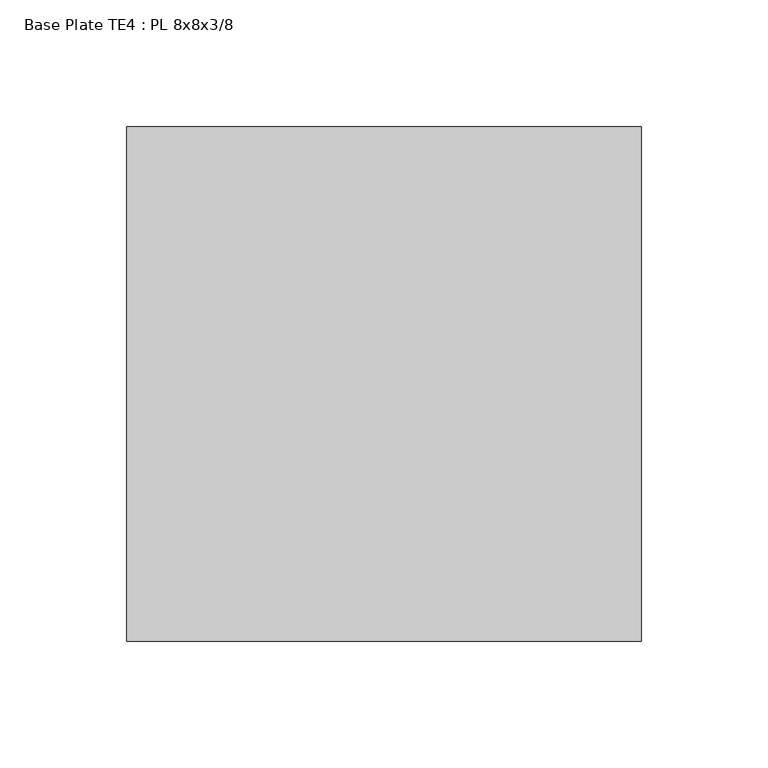
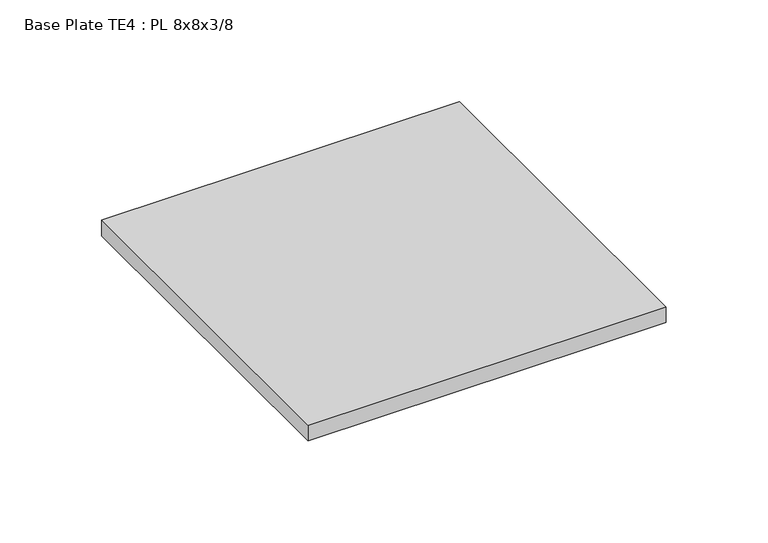
"""IFC4 building model written with IfcOpenShell, lengths in millimetres: proxy geometry, Base Plate TE4 : PL 8x8x3/8."""

import ifcopenshell
import ifcopenshell.guid

model = None  # the IFC model being written
_history = None  # IfcOwnerHistory: only IFC2X3 demands one
_inside = {}  # id of a spatial element -> (the spatial element, [elements in it])
_under = {}  # id of a project, library or spatial element -> (it, [spatial elements below it])
_declared = {}  # id of a project -> (the project, [libraries it declares])
_typed = {}  # id of a type object -> (the type object, [elements of that type])
_made_of = {}  # id of a material, layer set ... -> (it, [elements and type objects made of it])


def new_model(schema):
    """Start an empty IFC model of exactly this schema.

    Asked for "IFC4X3", IfcOpenShell would pick the latest addendum, in which some entities
    have other attributes; the version numbers below select the first issue.
    IFC2X3 requires an IfcOwnerHistory on every rooted entity: one is made here for all.
    """
    global model, _history
    if schema == "IFC4X3":
        model = ifcopenshell.file(schema_version=(4, 3, 0, 0))
    else:
        model = ifcopenshell.file(schema=schema)
    _inside.clear()
    _under.clear()
    _declared.clear()
    _typed.clear()
    _made_of.clear()
    _history = None
    if model.schema == "IFC2X3":
        org = make("IfcOrganization", Name="unknown")
        user = make(
            "IfcPersonAndOrganization",
            ThePerson=make("IfcPerson", FamilyName="unknown"),
            TheOrganization=org,
        )
        app = make(
            "IfcApplication",
            ApplicationDeveloper=org,
            Version="unknown",
            ApplicationFullName="unknown",
            ApplicationIdentifier="unknown",
        )
        _history = make(
            "IfcOwnerHistory",
            OwningUser=user,
            OwningApplication=app,
            ChangeAction="ADDED",
            CreationDate=0,
        )
    return model


def make(cls, **values):
    """One entity of the class cls with the attributes given. An attribute that is None is left unset."""
    return model.create_entity(
        cls, **{name: value for name, value in values.items() if value is not None}
    )


def rooted(cls, **values):
    """An entity with a GlobalId (a new one), such as an element, a storey or a relation."""
    return make(cls, GlobalId=ifcopenshell.guid.new(), OwnerHistory=_history, **values)


def si_unit(unit_type, name, prefix=None):
    """IfcSIUnit, for example si_unit("LENGTHUNIT", "METRE", prefix="MILLI")."""
    return make("IfcSIUnit", UnitType=unit_type, Prefix=prefix, Name=name)


def assignment(units):
    """IfcUnitAssignment: the units of a project."""
    return None if units is None else make("IfcUnitAssignment", Units=units)


def point(xyz):
    """IfcCartesianPoint."""
    return None if xyz is None else make("IfcCartesianPoint", Coordinates=xyz)


def direction(xyz):
    """IfcDirection."""
    return None if xyz is None else make("IfcDirection", DirectionRatios=xyz)


def frame(location, z_axis=None, x_axis=None):
    """IfcAxis2Placement3D, a coordinate frame: its origin and axes. An axis left out is left unset."""
    return make(
        "IfcAxis2Placement3D",
        Location=point(location),
        Axis=direction(z_axis),
        RefDirection=direction(x_axis),
    )


def origin():
    """The frame at (0, 0, 0) with its axes left unset."""
    return frame((0.0, 0.0, 0.0))


def place(relative_to, where):
    """IfcLocalPlacement: puts the frame where relative to a parent placement (None: the world)."""
    return make(
        "IfcLocalPlacement", PlacementRelTo=relative_to, RelativePlacement=where
    )


def context(
    kind, dimensions, precision=None, world=None, true_north=None, identifier=None
):
    """IfcGeometricRepresentationContext, for example the 3D "Model" context."""
    return make(
        "IfcGeometricRepresentationContext",
        ContextIdentifier=identifier,
        ContextType=kind,
        CoordinateSpaceDimension=dimensions,
        Precision=precision,
        WorldCoordinateSystem=world,
        TrueNorth=true_north,
    )


def project(units=None, contexts=None):
    """IfcProject with its units and contexts."""
    return rooted(
        "IfcProject",
        Name="project",
        RepresentationContexts=contexts,
        UnitsInContext=assignment(units),
    )


def spatial(cls, under=None, at=None, **own):
    """A site, building, storey or space (cls), placed at a placement, below another one or the project."""
    s = rooted(cls, ObjectPlacement=at, **own)
    if under is not None:
        _under.setdefault(under.id(), (under, []))[1].append(s)
    return s


def polyline(points):
    """IfcPolyline through the points."""
    return make("IfcPolyline", Points=[point(p) for p in points])


def outline(outer, holes=None, kind="AREA"):
    """IfcArbitraryClosedProfileDef: a profile drawn as a closed curve; with holes, ...WithVoids."""
    if holes is None:
        return make("IfcArbitraryClosedProfileDef", ProfileType=kind, OuterCurve=outer)
    return make(
        "IfcArbitraryProfileDefWithVoids",
        ProfileType=kind,
        OuterCurve=outer,
        InnerCurves=holes,
    )


def extrude(swept, where, along, depth):
    """IfcExtrudedAreaSolid: the profile swept, set in the frame where, extruded along a direction by depth."""
    return make(
        "IfcExtrudedAreaSolid",
        SweptArea=swept,
        Position=where,
        ExtrudedDirection=direction(along),
        Depth=depth,
    )


def shape(context_of_items, identifier, shape_type, items):
    """IfcShapeRepresentation: the items that make up one representation, for example the "Body"."""
    return make(
        "IfcShapeRepresentation",
        ContextOfItems=context_of_items,
        RepresentationIdentifier=identifier,
        RepresentationType=shape_type,
        Items=items,
    )


def source(mapping_origin, context_of_items, identifier, shape_type, items):
    """IfcRepresentationMap: a shape defined once, which mapped items show again and again."""
    return make(
        "IfcRepresentationMap",
        MappingOrigin=mapping_origin,
        MappedRepresentation=shape(context_of_items, identifier, shape_type, items),
    )


def transform(
    local_origin,
    x_axis=None,
    y_axis=None,
    z_axis=None,
    scale=None,
    scale2=None,
    scale3=None,
    uniform=True,
):
    """IfcCartesianTransformationOperator3D, or its non-uniform kind. x_axis, y_axis, z_axis: its Axis1, 2, 3."""
    if uniform:
        return make(
            "IfcCartesianTransformationOperator3D",
            Axis1=direction(x_axis),
            Axis2=direction(y_axis),
            LocalOrigin=point(local_origin),
            Scale=scale,
            Axis3=direction(z_axis),
        )
    return make(
        "IfcCartesianTransformationOperator3DnonUniform",
        Axis1=direction(x_axis),
        Axis2=direction(y_axis),
        LocalOrigin=point(local_origin),
        Scale=scale,
        Axis3=direction(z_axis),
        Scale2=scale2,
        Scale3=scale3,
    )


def mapped(mapping_source, mapping_target):
    """IfcMappedItem: shows the shape of a source again, moved by a transform."""
    return make(
        "IfcMappedItem", MappingSource=mapping_source, MappingTarget=mapping_target
    )


def made_of(thing, what):
    """Note that an element or type object is made of a material, layer set ...; save() writes the relation."""
    if what is not None:
        _made_of.setdefault(what.id(), (what, []))[1].append(thing)
    return thing


def element(
    cls,
    number,
    at=None,
    inside=None,
    cuts=None,
    type_object=None,
    material=None,
    context=None,
    identifier="Body",
    shape_type=None,
    held_by="IfcProductDefinitionShape",
    body=None,
    shapes=None,
    **own,
):
    """One element of the class cls, such as IfcWall. Its Tag is "e" and its number.

    at: its placement. inside: the storey or other place that contains it. cuts: it is an
    opening in that element (IfcRelVoidsElement). A single representation is given by context,
    identifier, shape_type and body (its items); several are given by shapes. held_by: the class
    of the entity that holds the representations. save() writes the other relations.
    """
    e = rooted(cls, Tag="e%d" % number, ObjectPlacement=at, **own)
    if body is not None:
        shapes = [shape(context, identifier, shape_type, body)]
    if shapes is not None:
        e.Representation = make(held_by, Representations=shapes)
    if inside is not None:
        _inside.setdefault(inside.id(), (inside, []))[1].append(e)
    if cuts is not None:
        rooted(
            "IfcRelVoidsElement", RelatingBuildingElement=cuts, RelatedOpeningElement=e
        )
    if type_object is not None:
        _typed.setdefault(type_object.id(), (type_object, []))[1].append(e)
    return made_of(e, material)


def aggregate(whole, parts):
    """IfcRelAggregates: a whole, such as a stair, and the parts it consists of."""
    return rooted("IfcRelAggregates", RelatingObject=whole, RelatedObjects=parts)


def save(model, path):
    """Write the relations noted so far, then the file.

    IfcRelAggregates (storeys below a building ...), IfcRelContainedInSpatialStructure (elements
    in a storey), IfcRelDefinesByType, IfcRelAssociatesMaterial and IfcRelDeclares: one each for
    every whole, place, type object, material and project.
    """
    for whole, parts in _under.values():
        aggregate(whole, parts)
    for where, things in _inside.values():
        rooted(
            "IfcRelContainedInSpatialStructure",
            RelatedElements=things,
            RelatingStructure=where,
        )
    for kind, things in _typed.values():
        rooted("IfcRelDefinesByType", RelatedObjects=things, RelatingType=kind)
    for what, things in _made_of.values():
        rooted("IfcRelAssociatesMaterial", RelatedObjects=things, RelatingMaterial=what)
    for by, libraries in _declared.values():
        rooted("IfcRelDeclares", RelatingContext=by, RelatedDefinitions=libraries)
    model.write(path)


def base_plate_te4_pl_8x8x3_8_c18328d5(model_context):
    return source(origin(), model_context, "Body", "SweptSolid", [
        extrude(outline(polyline([(590318.6599233, -536265.1913841), (590318.6599233, -536468.3913841), (590115.4599233, -536468.3913841), (590115.4599233, -536265.1913841), (590318.6599233, -536265.1913841)])), frame((0.0, 0.0, 19.05), z_axis=(0.0, 0.0, 1.0), x_axis=(1.0, 0.0, 0.0)), (0.0, 0.0, 1.0), 9.525),
    ])


if __name__ == "__main__":
    model = new_model("IFC4")
    model_context = context("Model", 3, world=origin())
    ifc_project = project(units=[si_unit("LENGTHUNIT", "METRE", prefix="MILLI")], contexts=[model_context])
    site = spatial("IfcSite", under=ifc_project)
    building = spatial("IfcBuilding", under=site)
    placement = place(None, origin())
    base_plate_te4_pl_8x8x3_8_shape = base_plate_te4_pl_8x8x3_8_c18328d5(model_context)
    element("IfcBuildingElementProxy", 1, Name="Base Plate TE4 : PL 8x8x3/8", ObjectType="Base Plate TE4 : PL 8x8x3/8", at=placement, inside=building, context=model_context, shape_type="MappedRepresentation", body=[
        mapped(base_plate_te4_pl_8x8x3_8_shape, transform((0.0, 0.0, 0.0), x_axis=(1.0, 0.0, 0.0), y_axis=(0.0, 1.0, 0.0), z_axis=(0.0, 0.0, 1.0))),
    ])
    save(model, "model.ifc")

# Revit data of these elements
# Element 1 (IfcBuildingElementProxy, "Base Plate TE4 : PL 8x8x3/8")
#   Materials on its faces: "GALV. STL BASE PLATE"
# Materials
#   "GALV. STL BASE PLATE": class "Generic", colour RGB 211 211 207, transparency 0, Cost = 0
